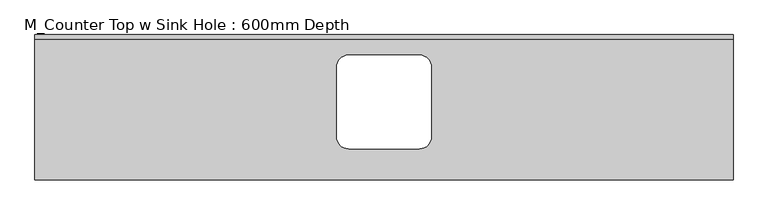
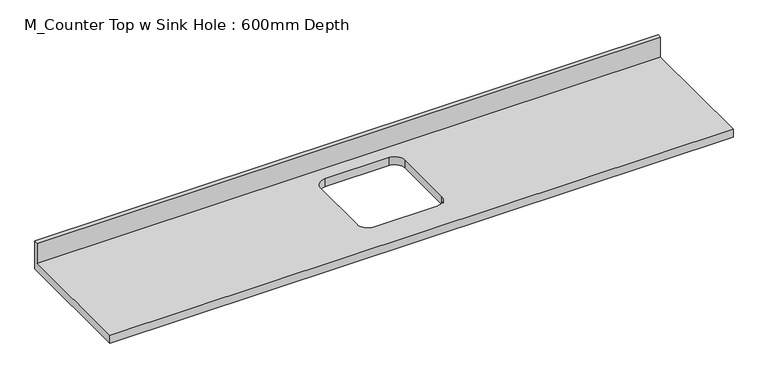
"""IFC4 building model written with IfcOpenShell, lengths in millimetres: furniture geometry, M_Counter Top w Sink Hole : 600mm Depth."""

from ifc_helpers import new_model, si_unit, frame, origin, place, context, project, spatial, polyline, circle_curve, source, transform, mapped, element, save
from ifc_brep_helpers import plane_surface, revolved_surface, advanced_brep


def m_counter_top_w_sink_hole_600mm_depth_b1bd1638(model_context):
    return source(origin(), model_context, "Body", "AdvancedBrep", [
        advanced_brep(
        [(-1200.4622951, -625.0, 900.0), (1799.5377049, -625.0, 900.0), (1799.5377049, -19.05, 900.0), (-1200.4622951, -19.05, 900.0), (147.2377049, -87.3, 900.0), (451.8377049, -87.3, 900.0), (502.6377049, -138.1, 900.0), (502.6377049, -439.9, 900.0), (451.8377049, -490.7, 900.0), (147.2377049, -490.7, 900.0), (96.4377049, -439.9, 900.0), (96.4377049, -138.1, 900.0), (1799.5377049, 0.0, 860.0), (1799.5377049, -625.0, 860.0), (-1200.4622951, -625.0, 860.0), (-1200.4622951, 0.0, 860.0), (451.8377049, -87.3, 860.0), (147.2377049, -87.3, 860.0), (96.4377049, -138.1, 860.0), (96.4377049, -439.9, 860.0), (147.2377049, -490.7, 860.0), (451.8377049, -490.7, 860.0), (502.6377049, -439.9, 860.0), (502.6377049, -138.1, 860.0), (-1200.4622951, 0.0, 1001.6), (1799.5377049, 0.0, 1001.6), (-1200.4622951, -19.05, 1001.6), (1799.5377049, -19.05, 1001.6)],
        [
            (0, 1),
            (1, 2),
            (2, 3),
            (3, 0),
            (4, 5),
            (5, 6, circle_curve(frame((451.8377049, -138.1, 900.0), z_axis=(0.0, 0.0, -1.0), x_axis=(1.0, 0.0, 0.0)), 50.8)),
            (6, 7),
            (7, 8, circle_curve(frame((451.8377049, -439.9, 900.0), z_axis=(0.0, 0.0, -1.0), x_axis=(1.0, 0.0, 0.0)), 50.8)),
            (8, 9),
            (9, 10, circle_curve(frame((147.2377049, -439.9, 900.0), z_axis=(0.0, 0.0, -1.0), x_axis=(1.0, 0.0, 0.0)), 50.8)),
            (10, 11),
            (11, 4, circle_curve(frame((147.2377049, -138.1, 900.0), z_axis=(0.0, 0.0, -1.0), x_axis=(1.0, 0.0, 0.0)), 50.8)),
            (12, 13),
            (13, 14),
            (14, 15),
            (15, 12),
            (16, 17),
            (17, 18, circle_curve(frame((147.2377049, -138.1, 860.0), z_axis=(0.0, 0.0, 1.0), x_axis=(1.0, 0.0, 0.0)), 50.8)),
            (18, 19),
            (19, 20, circle_curve(frame((147.2377049, -439.9, 860.0), z_axis=(0.0, 0.0, 1.0), x_axis=(1.0, 0.0, 0.0)), 50.8)),
            (20, 21),
            (21, 22, circle_curve(frame((451.8377049, -439.9, 860.0), z_axis=(0.0, 0.0, 1.0), x_axis=(1.0, 0.0, 0.0)), 50.8)),
            (22, 23),
            (23, 16, circle_curve(frame((451.8377049, -138.1, 860.0), z_axis=(0.0, 0.0, 1.0), x_axis=(1.0, 0.0, 0.0)), 50.8)),
            (15, 24),
            (24, 25),
            (25, 12),
            (14, 0),
            (3, 26),
            (26, 24),
            (13, 1),
            (25, 27),
            (27, 2),
            (26, 27),
            (4, 17),
            (16, 5),
            (11, 18),
            (10, 19),
            (9, 20),
            (8, 21),
            (7, 22),
            (6, 23),
        ],
        [
            plane_surface(frame((-1200.4622951, 0.0, 900.0), z_axis=(0.0, 0.0, 1.0), x_axis=(-1.0, 0.0, 0.0))),
            plane_surface(frame((-1200.4622951, 0.0, 860.0), z_axis=(0.0, 0.0, -1.0), x_axis=(1.0, 0.0, 0.0))),
            plane_surface(frame((1799.5377049, 0.0, 900.0), z_axis=(0.0, 1.0, 0.0), x_axis=(0.0, 0.0, -1.0))),
            plane_surface(frame((-1200.4622951, 0.0, 900.0), z_axis=(-1.0, 0.0, 0.0), x_axis=(0.0, 0.0, -1.0))),
            plane_surface(frame((-1200.4622951, -625.0, 900.0), z_axis=(0.0, -1.0, 0.0), x_axis=(0.0, 0.0, -1.0))),
            plane_surface(frame((1799.5377049, -625.0, 900.0), z_axis=(1.0, 0.0, 0.0), x_axis=(0.0, 0.0, -1.0))),
            plane_surface(frame((-1200.4622951, 0.0, 1001.6), z_axis=(0.0, 0.0, 1.0), x_axis=(0.0, -1.0, 0.0))),
            plane_surface(frame((-1200.4622951, -19.05, 1001.6), z_axis=(0.0, -1.0, 0.0), x_axis=(0.0, 0.0, -1.0))),
            plane_surface(frame((451.8377049, -87.3, 900.0), z_axis=(0.0, -1.0, 0.0), x_axis=(0.0, 0.0, -1.0))),
            revolved_surface(polyline([(198.0377049, -138.1, 900.0), (198.0377049, -138.1, 860.0)]), (147.2377049, -138.1, 860.0), (0.0, 0.0, 1.0)),
            plane_surface(frame((96.4377049, -138.1, 900.0), z_axis=(1.0, 0.0, 0.0), x_axis=(0.0, 0.0, -1.0))),
            revolved_surface(polyline([(198.0377049, -439.9, 900.0), (198.0377049, -439.9, 860.0)]), (147.2377049, -439.9, 860.0), (0.0, 0.0, 1.0)),
            plane_surface(frame((147.2377049, -490.7, 900.0), z_axis=(0.0, 1.0, 0.0), x_axis=(0.0, 0.0, -1.0))),
            revolved_surface(polyline([(502.6377049, -439.9, 900.0), (502.6377049, -439.9, 860.0)]), (451.8377049, -439.9, 860.0), (0.0, 0.0, 1.0)),
            plane_surface(frame((502.6377049, -439.9, 900.0), z_axis=(-1.0, 0.0, 0.0), x_axis=(0.0, 0.0, -1.0))),
            revolved_surface(polyline([(502.6377049, -138.1, 900.0), (502.6377049, -138.1, 860.0)]), (451.8377049, -138.1, 860.0), (0.0, 0.0, 1.0)),
        ],
        [
            (0, [[1, 2, 3, 4], [5, 6, 7, 8, 9, 10, 11, 12]]),
            (1, [[13, 14, 15, 16], [17, 18, 19, 20, 21, 22, 23, 24]]),
            (2, [[-16, 25, 26, 27]]),
            (3, [[-15, 28, -4, 29, 30, -25]]),
            (4, [[-1, -28, -14, 31]]),
            (5, [[-13, -27, 32, 33, -2, -31]]),
            (6, [[-30, 34, -32, -26]]),
            (7, [[-34, -29, -3, -33]]),
            (8, [[35, -17, 36, -5]]),
            (9, [[-35, -12, 37, -18]]),
            (10, [[-37, -11, 38, -19]]),
            (11, [[-38, -10, 39, -20]]),
            (12, [[-39, -9, 40, -21]]),
            (13, [[-40, -8, 41, -22]]),
            (14, [[-41, -7, 42, -23]]),
            (15, [[-36, -24, -42, -6]]),
        ],
    ),
    ])


if __name__ == "__main__":
    model = new_model("IFC4")
    model_context = context("Model", 3, world=origin())
    ifc_project = project(units=[si_unit("LENGTHUNIT", "METRE", prefix="MILLI")], contexts=[model_context])
    site = spatial("IfcSite", under=ifc_project)
    building = spatial("IfcBuilding", under=site)
    placement = place(None, origin())
    m_counter_top_w_sink_hole_600mm_depth_shape = m_counter_top_w_sink_hole_600mm_depth_b1bd1638(model_context)
    element("IfcFurniture", 1, ObjectType="M_Counter Top w Sink Hole : 600mm Depth", at=placement, inside=building, context=model_context, shape_type="MappedRepresentation", body=[
        mapped(m_counter_top_w_sink_hole_600mm_depth_shape, transform((0.0, 0.0, 0.0), x_axis=(1.0, 0.0, 0.0), y_axis=(0.0, 1.0, 0.0), z_axis=(0.0, 0.0, 1.0))),
    ])
    save(model, "model.ifc")

# Revit data of these elements
# Type "M_Counter Top w Sink Hole : 600mm Depth"
#   Manufacturer = "Manufacturer"
#   Finish = "Finish"
#   Construction Type = "Construction Type"
#   AccessibilityPerformance = "AccessibilityPerformance"
#   CodePerformance = "CodePerformance"
#   Area = "Area"
#   Color = "Color"
#   Constituents = "Constituents"
#   Features = "Features"
#   Finish = "Finish"
#   Grade = "Grade"
#   Material = "Material"
#   ModelReference = "ModelReference"
#   NominalHeight = "NominalHeight"
#   NominalLength = "NominalLength"
#   NominalWidth = "NominalWidth"
#   ProductionYear = "ProductionYear"
#   Reference = "Reference"
#   Shape = "Shape"
#   Size = "Size"
#   SustainabilityPerformance = "SustainabilityPerformance"
#   WarrantyDescription = "WarrantyDescription"
#   WarrantyDurationLabor = "WarrantyDurationLabor"
#   WarrantyDurationParts = "WarrantyDurationParts"
#   WarrantyGuarantorLabor = "WarrantyGuarantorLabor"
#   WarrantyGuarantorParts = "WarrantyGuarantorParts"
#   ExpectedLife = "ExpectedLife"
#   ReplacementCost = "ReplacementCost"
#   AssetAccountingType = "FIXED"
#   ModelLabel = "ModelLabel"
#   Counter Thickness = 0.040 m
#   Depth = 0.625 m
#   Height = 0.900 m
#   Length [instance default] = 2.500 m
#   Sink Location [instance default] = 1.200 m
#   Sink Location To Wall [instance default] = 0.100 m
#   Sink Opening Depth [instance default] = 0.378 m
#   Sink Opening Width [instance default] = 0.587 m
#   Counter Top Material = none
# Element 1 (IfcFurniture, "M_Counter Top w Sink Hole : 600mm Depth")
#   Length = 3.000 m
#   Sink Location = 1.500 m
#   Sink Opening Width = 0.3808 m
#   Materials on its faces: "Counter Top"
# Materials
#   "Counter Top": class "Wood", colour RGB 226 177 128, transparency 0
